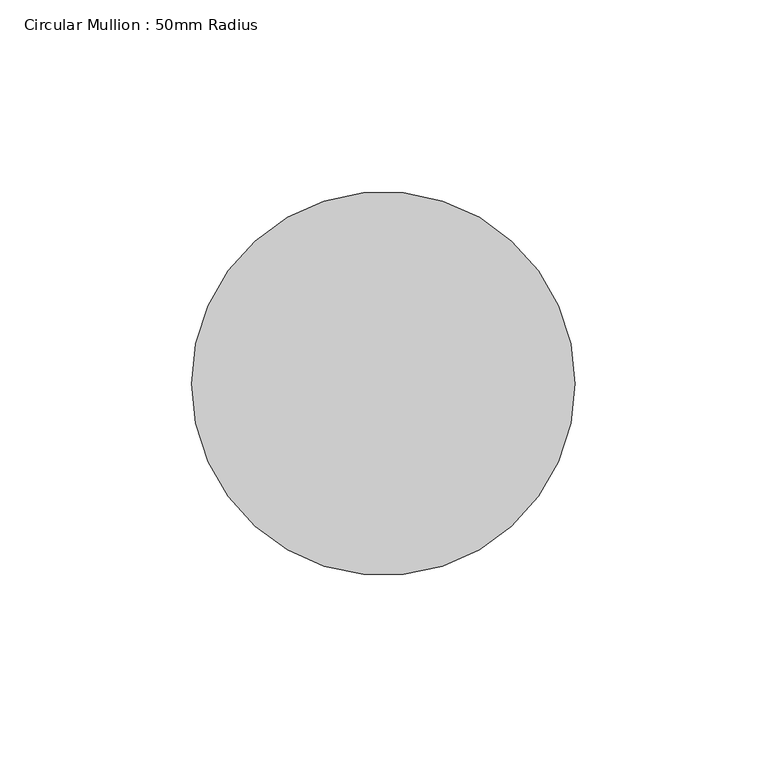
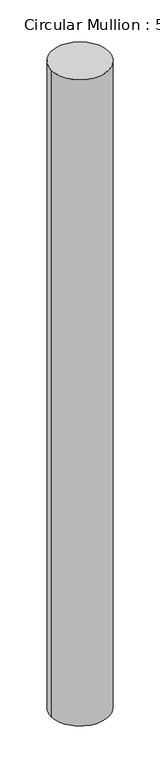
"""IFC4 building model written with IfcOpenShell, lengths in millimetres: member geometry, Circular Mullion : 50mm Radius."""

from ifc_helpers import new_model, si_unit, point, frame, origin, origin_2d, place, context, project, spatial, circle_curve, trimmed, segment, composite_curve, outline, extrude, source, transform, mapped, element, save


def circular_mullion_50mm_radius_a3e757a6(model_context):
    return source(origin(), model_context, "Body", "SweptSolid", [
        extrude(outline(composite_curve([segment(trimmed(circle_curve(origin_2d(), 50.0), [point((50.0, 0.0))], [point((-50.0, 0.0))], False, "CARTESIAN"), True, "CONTINUOUS"), segment(trimmed(circle_curve(origin_2d(), 50.0), [point((-50.0, 0.0))], [point((50.0, 0.0))], False, "CARTESIAN"), True, "CONTINUOUS")], self_intersect=False)), frame((0.0, 0.0, -1191.7229322), z_axis=(0.0, 0.0, 1.0), x_axis=(1.0, 0.0, 0.0)), (0.0, 0.0, 1.0), 1191.7229322),
    ])


if __name__ == "__main__":
    model = new_model("IFC4")
    model_context = context("Model", 3, world=origin())
    ifc_project = project(units=[si_unit("LENGTHUNIT", "METRE", prefix="MILLI")], contexts=[model_context])
    site = spatial("IfcSite", under=ifc_project)
    building = spatial("IfcBuilding", under=site)
    placement = place(None, origin())
    circular_mullion_50mm_radius_shape = circular_mullion_50mm_radius_a3e757a6(model_context)
    element("IfcMember", 1, ObjectType="Circular Mullion : 50mm Radius", at=placement, inside=building, context=model_context, shape_type="MappedRepresentation", body=[
        mapped(circular_mullion_50mm_radius_shape, transform((0.0, 0.0, 0.0), x_axis=(1.0, 0.0, 0.0), y_axis=(0.0, 1.0, 0.0), z_axis=(0.0, 0.0, 1.0))),
    ])
    save(model, "model.ifc")

# Revit data of these elements
# Type "Circular Mullion : 50mm Radius"
#   built-in parameter 1007350 = 0.164042 (stored number, unit not read)
# Element 1 (IfcMember, "Circular Mullion : 50mm Radius")
#   Materials on its faces: "Aluminium"
# Materials
#   "Aluminium": class "Metal", colour RGB 247 247 247, transparency 0, Description = "Aluminium 6061", Cost = 0
